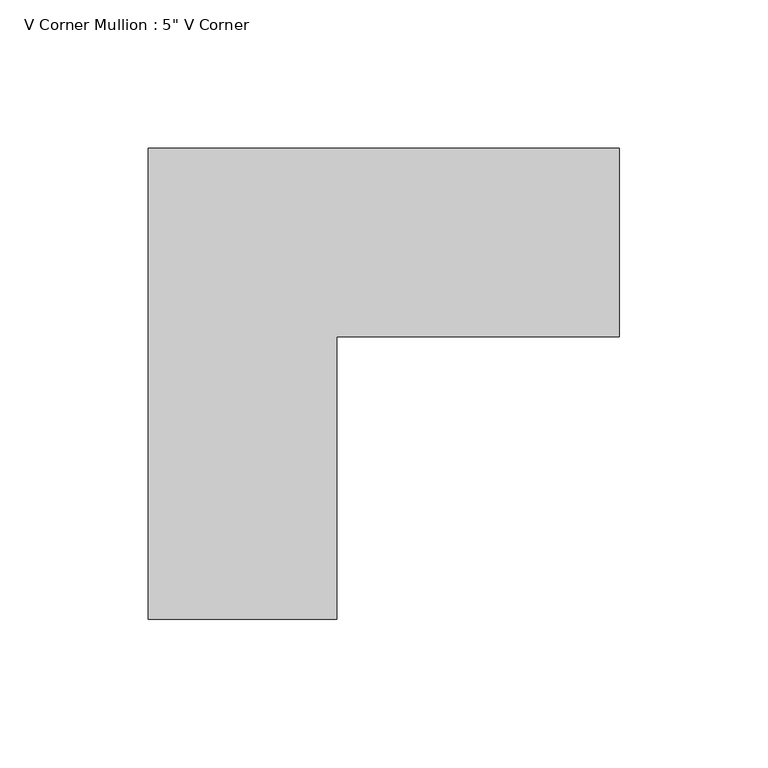
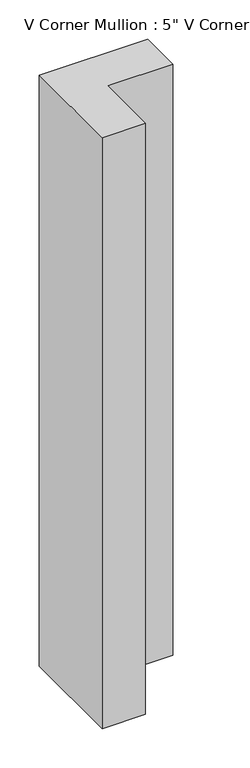
"""IFC4 building model written with IfcOpenShell, lengths in millimetres: member geometry."""

from ifc_helpers import new_model, si_unit, frame, origin, place, context, project, spatial, polyline, outline, extrude, source, transform, mapped, element, save


def member_9ba7d3b0(model_context):
    return source(origin(), model_context, "Body", "SweptSolid", [
        extrude(outline(polyline([(63.5, 31.75), (-31.75, 31.75), (-31.75, -63.5), (-95.25, -63.5), (-95.25, 95.25), (63.5, 95.25), (63.5, 31.75)])), frame((0.0, 0.0, -914.4), z_axis=(0.0, 0.0, 1.0), x_axis=(1.0, 0.0, 0.0)), (0.0, 0.0, 1.0), 914.4),
    ])


if __name__ == "__main__":
    model = new_model("IFC4")
    model_context = context("Model", 3, world=origin())
    ifc_project = project(units=[si_unit("LENGTHUNIT", "METRE", prefix="MILLI")], contexts=[model_context])
    site = spatial("IfcSite", under=ifc_project)
    building = spatial("IfcBuilding", under=site)
    placement = place(None, origin())
    member_shape = member_9ba7d3b0(model_context)
    element("IfcMember", 1, ObjectType="V Corner Mullion : 5\" V Corner", at=placement, inside=building, context=model_context, shape_type="MappedRepresentation", body=[
        mapped(member_shape, transform((0.0, 0.0, 0.0), x_axis=(1.0, 0.0, 0.0), y_axis=(0.0, 1.0, 0.0), z_axis=(0.0, 0.0, 1.0))),
    ])
    save(model, "model.ifc")

# Revit data of these elements
# Type "V Corner Mullion : 5\" V Corner"
#   built-in parameter 1007355 = 0.416667 (stored number, unit not read)
#   built-in parameter 1007354 = 0.416667 (stored number, unit not read)
#   built-in parameter 1007304 = 0.208333 (stored number, unit not read)
# Element 1 (IfcMember, "V Corner Mullion : 5\" V Corner")
#   Materials on its faces: "Aluminum"
# Materials
#   "Aluminum": class "Metal", colour RGB 244 245 246, transparency 0, Description = "Aluminum 6061", Cost = 0
